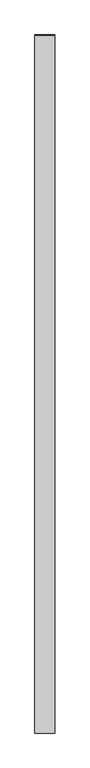
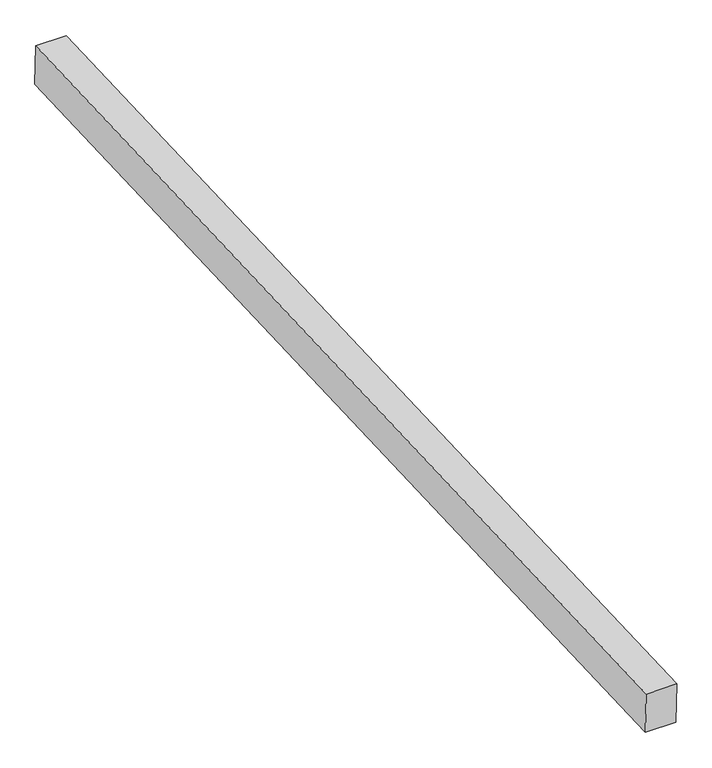
"""IFC4 building model written with IfcOpenShell, lengths in millimetres: proxy geometry, Generic Models 7:Generic Models 1:8:Generic Models 1:8 : Generic Models 7:Generic Models 1:337419:23 : Generic Models 7:Generic Models 1:8:Generic Models 1:8 : Generic Models 7:Generic Models 1:337419:315935."""

import ifcopenshell
import ifcopenshell.guid

model = None  # the IFC model being written
_history = None  # IfcOwnerHistory: only IFC2X3 demands one
_inside = {}  # id of a spatial element -> (the spatial element, [elements in it])
_under = {}  # id of a project, library or spatial element -> (it, [spatial elements below it])
_declared = {}  # id of a project -> (the project, [libraries it declares])
_typed = {}  # id of a type object -> (the type object, [elements of that type])
_made_of = {}  # id of a material, layer set ... -> (it, [elements and type objects made of it])


def new_model(schema):
    """Start an empty IFC model of exactly this schema.

    Asked for "IFC4X3", IfcOpenShell would pick the latest addendum, in which some entities
    have other attributes; the version numbers below select the first issue.
    IFC2X3 requires an IfcOwnerHistory on every rooted entity: one is made here for all.
    """
    global model, _history
    if schema == "IFC4X3":
        model = ifcopenshell.file(schema_version=(4, 3, 0, 0))
    else:
        model = ifcopenshell.file(schema=schema)
    _inside.clear()
    _under.clear()
    _declared.clear()
    _typed.clear()
    _made_of.clear()
    _history = None
    if model.schema == "IFC2X3":
        org = make("IfcOrganization", Name="unknown")
        user = make(
            "IfcPersonAndOrganization",
            ThePerson=make("IfcPerson", FamilyName="unknown"),
            TheOrganization=org,
        )
        app = make(
            "IfcApplication",
            ApplicationDeveloper=org,
            Version="unknown",
            ApplicationFullName="unknown",
            ApplicationIdentifier="unknown",
        )
        _history = make(
            "IfcOwnerHistory",
            OwningUser=user,
            OwningApplication=app,
            ChangeAction="ADDED",
            CreationDate=0,
        )
    return model


def make(cls, **values):
    """One entity of the class cls with the attributes given. An attribute that is None is left unset."""
    return model.create_entity(
        cls, **{name: value for name, value in values.items() if value is not None}
    )


def rooted(cls, **values):
    """An entity with a GlobalId (a new one), such as an element, a storey or a relation."""
    return make(cls, GlobalId=ifcopenshell.guid.new(), OwnerHistory=_history, **values)


def si_unit(unit_type, name, prefix=None):
    """IfcSIUnit, for example si_unit("LENGTHUNIT", "METRE", prefix="MILLI")."""
    return make("IfcSIUnit", UnitType=unit_type, Prefix=prefix, Name=name)


def assignment(units):
    """IfcUnitAssignment: the units of a project."""
    return None if units is None else make("IfcUnitAssignment", Units=units)


def point(xyz):
    """IfcCartesianPoint."""
    return None if xyz is None else make("IfcCartesianPoint", Coordinates=xyz)


def direction(xyz):
    """IfcDirection."""
    return None if xyz is None else make("IfcDirection", DirectionRatios=xyz)


def frame(location, z_axis=None, x_axis=None):
    """IfcAxis2Placement3D, a coordinate frame: its origin and axes. An axis left out is left unset."""
    return make(
        "IfcAxis2Placement3D",
        Location=point(location),
        Axis=direction(z_axis),
        RefDirection=direction(x_axis),
    )


def origin():
    """The frame at (0, 0, 0) with its axes left unset."""
    return frame((0.0, 0.0, 0.0))


def place(relative_to, where):
    """IfcLocalPlacement: puts the frame where relative to a parent placement (None: the world)."""
    return make(
        "IfcLocalPlacement", PlacementRelTo=relative_to, RelativePlacement=where
    )


def context(
    kind, dimensions, precision=None, world=None, true_north=None, identifier=None
):
    """IfcGeometricRepresentationContext, for example the 3D "Model" context."""
    return make(
        "IfcGeometricRepresentationContext",
        ContextIdentifier=identifier,
        ContextType=kind,
        CoordinateSpaceDimension=dimensions,
        Precision=precision,
        WorldCoordinateSystem=world,
        TrueNorth=true_north,
    )


def project(units=None, contexts=None):
    """IfcProject with its units and contexts."""
    return rooted(
        "IfcProject",
        Name="project",
        RepresentationContexts=contexts,
        UnitsInContext=assignment(units),
    )


def spatial(cls, under=None, at=None, **own):
    """A site, building, storey or space (cls), placed at a placement, below another one or the project."""
    s = rooted(cls, ObjectPlacement=at, **own)
    if under is not None:
        _under.setdefault(under.id(), (under, []))[1].append(s)
    return s


def polyline(points):
    """IfcPolyline through the points."""
    return make("IfcPolyline", Points=[point(p) for p in points])


def outline(outer, holes=None, kind="AREA"):
    """IfcArbitraryClosedProfileDef: a profile drawn as a closed curve; with holes, ...WithVoids."""
    if holes is None:
        return make("IfcArbitraryClosedProfileDef", ProfileType=kind, OuterCurve=outer)
    return make(
        "IfcArbitraryProfileDefWithVoids",
        ProfileType=kind,
        OuterCurve=outer,
        InnerCurves=holes,
    )


def extrude(swept, where, along, depth):
    """IfcExtrudedAreaSolid: the profile swept, set in the frame where, extruded along a direction by depth."""
    return make(
        "IfcExtrudedAreaSolid",
        SweptArea=swept,
        Position=where,
        ExtrudedDirection=direction(along),
        Depth=depth,
    )


def shape(context_of_items, identifier, shape_type, items):
    """IfcShapeRepresentation: the items that make up one representation, for example the "Body"."""
    return make(
        "IfcShapeRepresentation",
        ContextOfItems=context_of_items,
        RepresentationIdentifier=identifier,
        RepresentationType=shape_type,
        Items=items,
    )


def source(mapping_origin, context_of_items, identifier, shape_type, items):
    """IfcRepresentationMap: a shape defined once, which mapped items show again and again."""
    return make(
        "IfcRepresentationMap",
        MappingOrigin=mapping_origin,
        MappedRepresentation=shape(context_of_items, identifier, shape_type, items),
    )


def transform(
    local_origin,
    x_axis=None,
    y_axis=None,
    z_axis=None,
    scale=None,
    scale2=None,
    scale3=None,
    uniform=True,
):
    """IfcCartesianTransformationOperator3D, or its non-uniform kind. x_axis, y_axis, z_axis: its Axis1, 2, 3."""
    if uniform:
        return make(
            "IfcCartesianTransformationOperator3D",
            Axis1=direction(x_axis),
            Axis2=direction(y_axis),
            LocalOrigin=point(local_origin),
            Scale=scale,
            Axis3=direction(z_axis),
        )
    return make(
        "IfcCartesianTransformationOperator3DnonUniform",
        Axis1=direction(x_axis),
        Axis2=direction(y_axis),
        LocalOrigin=point(local_origin),
        Scale=scale,
        Axis3=direction(z_axis),
        Scale2=scale2,
        Scale3=scale3,
    )


def mapped(mapping_source, mapping_target):
    """IfcMappedItem: shows the shape of a source again, moved by a transform."""
    return make(
        "IfcMappedItem", MappingSource=mapping_source, MappingTarget=mapping_target
    )


def made_of(thing, what):
    """Note that an element or type object is made of a material, layer set ...; save() writes the relation."""
    if what is not None:
        _made_of.setdefault(what.id(), (what, []))[1].append(thing)
    return thing


def element(
    cls,
    number,
    at=None,
    inside=None,
    cuts=None,
    type_object=None,
    material=None,
    context=None,
    identifier="Body",
    shape_type=None,
    held_by="IfcProductDefinitionShape",
    body=None,
    shapes=None,
    **own,
):
    """One element of the class cls, such as IfcWall. Its Tag is "e" and its number.

    at: its placement. inside: the storey or other place that contains it. cuts: it is an
    opening in that element (IfcRelVoidsElement). A single representation is given by context,
    identifier, shape_type and body (its items); several are given by shapes. held_by: the class
    of the entity that holds the representations. save() writes the other relations.
    """
    e = rooted(cls, Tag="e%d" % number, ObjectPlacement=at, **own)
    if body is not None:
        shapes = [shape(context, identifier, shape_type, body)]
    if shapes is not None:
        e.Representation = make(held_by, Representations=shapes)
    if inside is not None:
        _inside.setdefault(inside.id(), (inside, []))[1].append(e)
    if cuts is not None:
        rooted(
            "IfcRelVoidsElement", RelatingBuildingElement=cuts, RelatedOpeningElement=e
        )
    if type_object is not None:
        _typed.setdefault(type_object.id(), (type_object, []))[1].append(e)
    return made_of(e, material)


def aggregate(whole, parts):
    """IfcRelAggregates: a whole, such as a stair, and the parts it consists of."""
    return rooted("IfcRelAggregates", RelatingObject=whole, RelatedObjects=parts)


def save(model, path):
    """Write the relations noted so far, then the file.

    IfcRelAggregates (storeys below a building ...), IfcRelContainedInSpatialStructure (elements
    in a storey), IfcRelDefinesByType, IfcRelAssociatesMaterial and IfcRelDeclares: one each for
    every whole, place, type object, material and project.
    """
    for whole, parts in _under.values():
        aggregate(whole, parts)
    for where, things in _inside.values():
        rooted(
            "IfcRelContainedInSpatialStructure",
            RelatedElements=things,
            RelatingStructure=where,
        )
    for kind, things in _typed.values():
        rooted("IfcRelDefinesByType", RelatedObjects=things, RelatingType=kind)
    for what, things in _made_of.values():
        rooted("IfcRelAssociatesMaterial", RelatedObjects=things, RelatingMaterial=what)
    for by, libraries in _declared.values():
        rooted("IfcRelDeclares", RelatingContext=by, RelatedDefinitions=libraries)
    model.write(path)


def generic_models_ef17e683(model_context):
    return source(origin(), model_context, "Body", "SweptSolid", [
        extrude(outline(polyline([(-569809.5331551, 8697.9424054), (-564936.6102609, 8900.9808594), (-564929.0433392, 8710.6308549), (-569801.6025364, 8507.607555), (-569809.5331551, 8697.9424054)])), frame((593665.0617243, 0.0, 0.0), z_axis=(1.0, 0.0, 0.0), x_axis=(0.0, 1.0, 0.0)), (0.0, 0.0, 1.0), 139.7),
    ])


if __name__ == "__main__":
    model = new_model("IFC4")
    model_context = context("Model", 3, world=origin())
    ifc_project = project(units=[si_unit("LENGTHUNIT", "METRE", prefix="MILLI")], contexts=[model_context])
    site = spatial("IfcSite", under=ifc_project)
    building = spatial("IfcBuilding", under=site)
    placement = place(None, origin())
    generic_models_shape = generic_models_ef17e683(model_context)
    element("IfcBuildingElementProxy", 1, Name="Generic Models 7:Generic Models 1:8:Generic Models 1:8 : Generic Models 7:Generic Models 1:337419:23 : Generic Models 7:Generic Models 1:8:Generic Models 1:8 : Generic Models 7:Generic Models 1:337419:315935", ObjectType="Generic Models 7:Generic Models 1:8:Generic Models 1:8 : Generic Models 7:Generic Models 1:337419:23 : Generic Models 7:Generic Models 1:8:Generic Models 1:8 : Generic Models 7:Generic Models 1:337419:315935", at=placement, inside=building, context=model_context, shape_type="MappedRepresentation", body=[
        mapped(generic_models_shape, transform((0.0, 0.0, 0.0), x_axis=(1.0, 0.0, 0.0), y_axis=(0.0, 1.0, 0.0), z_axis=(0.0, 0.0, 1.0))),
    ])
    save(model, "model.ifc")

# Revit data of these elements
# Type "Generic Models 7:Generic Models 1:8:Generic Models 1:8 : Generic Models 7:Generic Models 1:337419:23 : Generic Models 7:Generic Models 1:8:Generic Models 1:8 : Generic Models 7:Generic Models 1:337419:315935"
#   NameOverride = "Generic Models 7:Generic Models 1:8:Generic Models 1:8 : Generic Models 7:Generic Models 1:337419:315935"
#   ObjectTypeOverride = "Generic Models 1:8 : Generic Models 7:Generic Models 1:337419"
#   Reference = "Generic Models 1"
#   Tag = "315935"
# Element 1 (IfcBuildingElementProxy, "Generic Models 7:Generic Models 1:8:Generic Models 1:8 : Generic Models 7:Generic Models 1:337419:23 : Generic Models 7:Generic Models 1:8:Generic Models 1:8 : Generic Models 7:Generic Models 1:337419:315935")
#   Materials on its faces: "5 1/2\" X 7 1/2\" EXTERIOR GRADE GLULAM BEAMS"
# Materials
#   "5 1/2\" X 7 1/2\" EXTERIOR GRADE GLULAM BEAMS": class "Wood", colour RGB 183 134 68, transparency 0, Keynote = "M06181300.01", Description = "Pinus Echinata", Cost = 0
